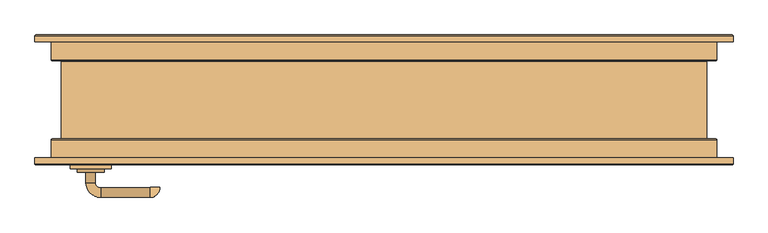
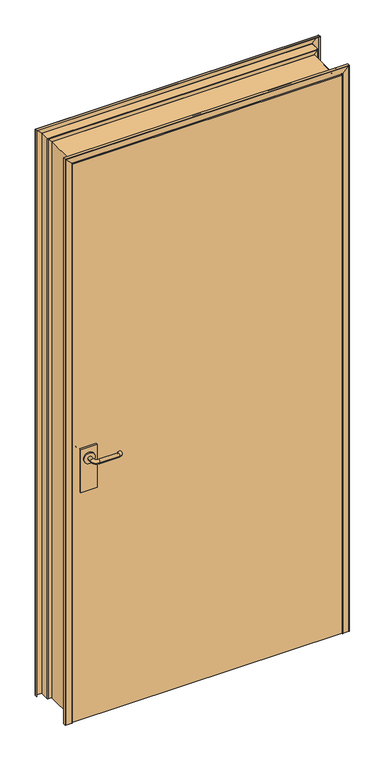
"""IFC4 building model written with IfcOpenShell, lengths in millimetres: door geometry, Porta Simples de Abrir : 90x210cm - Marco Metálico."""

from ifc_helpers import new_model, si_unit, point, frame, frame_2d, origin, place, context, project, spatial, polyline, circle_curve, ellipse_curve, trimmed, segment, composite_curve, outline, extrude, source, transform, mapped, element, save
from ifc_brep_helpers import plane_surface, cylinder_surface, revolved_surface, advanced_brep


def door_5cabed0b(model_context):
    return source(origin(), model_context, "Body", "SolidModel", [
        extrude(outline(composite_curve([segment(trimmed(circle_curve(frame_2d((1050.0, -432.0)), 20.0), [point((1050.0, -452.0))], [point((1050.0, -412.0))], False, "CARTESIAN"), True, "CONTINUOUS"), segment(trimmed(circle_curve(frame_2d((1050.0, -432.0)), 20.0), [point((1050.0, -412.0))], [point((1050.0, -452.0))], False, "CARTESIAN"), True, "CONTINUOUS")], self_intersect=False)), frame((0.0, -54.6, 0.0), z_axis=(0.0, 1.0, 0.0), x_axis=(0.0, 0.0, 1.0)), (0.0, 0.0, 1.0), 4.5929895),
        advanced_brep(
        [(-425.0, -50.0070105, 1050.0), (-439.0, -50.0070105, 1050.0), (-425.0, -34.6, 1050.0), (-439.0, -34.6, 1050.0), (-417.0, -12.6, 1050.0), (-417.0, -26.6, 1050.0), (-345.0, -26.6, 1050.0), (-345.0, -12.6, 1050.0), (-344.0, -27.6, 1050.0), (-330.0, -27.6, 1050.0)],
        [
            (0, 1, circle_curve(frame((-432.0, -50.0070105, 1050.0), z_axis=(0.0, -1.0, 0.0), x_axis=(-1.0, 0.0, 0.0)), 7.0)),
            (1, 0, circle_curve(frame((-432.0, -50.0070105, 1050.0), z_axis=(0.0, -1.0, 0.0), x_axis=(-1.0, 0.0, 0.0)), 7.0)),
            (0, 2),
            (2, 3, circle_curve(frame((-432.0, -34.6, 1050.0), z_axis=(0.0, -1.0, 0.0), x_axis=(-1.0, 0.0, 0.0)), 7.0)),
            (3, 1),
            (3, 2, circle_curve(frame((-432.0, -34.6, 1050.0), z_axis=(0.0, -1.0, 0.0), x_axis=(-1.0, 0.0, 0.0)), 7.0)),
            (4, 3, circle_curve(frame((-417.0, -34.6, 1050.0), z_axis=(0.0, 0.0, 1.0), x_axis=(-1.0, 0.0, 0.0)), 22.0)),
            (2, 5, circle_curve(frame((-417.0, -34.6, 1050.0), z_axis=(0.0, 0.0, -1.0), x_axis=(-1.0, 0.0, 0.0)), 8.0)),
            (5, 4, circle_curve(frame((-417.0, -19.6, 1050.0), z_axis=(-1.0, 0.0, 0.0), x_axis=(0.0, 1.0, 0.0)), 7.0)),
            (4, 5, circle_curve(frame((-417.0, -19.6, 1050.0), z_axis=(-1.0, 0.0, 0.0), x_axis=(0.0, 1.0, 0.0)), 7.0)),
            (5, 6),
            (6, 7, circle_curve(frame((-345.0, -19.6, 1050.0), z_axis=(-1.0, 0.0, 0.0), x_axis=(0.0, 1.0, 0.0)), 7.0)),
            (7, 4),
            (7, 6, circle_curve(frame((-345.0, -19.6, 1050.0), z_axis=(-1.0, 0.0, 0.0), x_axis=(0.0, 1.0, 0.0)), 7.0)),
            (8, 9, circle_curve(frame((-337.0, -27.6, 1050.0), z_axis=(0.0, -1.0, 0.0), x_axis=(1.0, 0.0, 0.0)), 7.0)),
            (9, 8, circle_curve(frame((-337.0, -27.6, 1050.0), z_axis=(0.0, -1.0, 0.0), x_axis=(1.0, 0.0, 0.0)), 7.0)),
            (9, 7, circle_curve(frame((-345.0, -27.6, 1050.0), z_axis=(0.0, 0.0, 1.0), x_axis=(0.0, 1.0, 0.0)), 15.0)),
            (6, 8, circle_curve(frame((-345.0, -27.6, 1050.0), z_axis=(0.0, 0.0, -1.0), x_axis=(0.0, 1.0, 0.0)), 1.0)),
        ],
        [
            plane_surface(frame((-432.0, -50.0070105, 1050.0), z_axis=(0.0, -1.0, 0.0), x_axis=(0.0, 0.0, 1.0))),
            cylinder_surface(frame((-432.0, -50.0070105, 1050.0), z_axis=(0.0, -1.0, 0.0), x_axis=(-1.0, 0.0, 0.0)), 7.0),
            revolved_surface(trimmed(ellipse_curve(frame((-432.0, -34.6, 1050.0), z_axis=(0.0, -1.0, 0.0), x_axis=(-1.0, 0.0, 0.0)), 7.0, 7.0), [point((-425.0, -34.6, 1050.0))], [point((-439.0, -34.6, 1050.0))], True, "CARTESIAN"), (-417.0, -34.6, 1050.0), (0.0, 0.0, -1.0)),
            revolved_surface(trimmed(ellipse_curve(frame((-432.0, -34.6, 1050.0), z_axis=(0.0, -1.0, 0.0), x_axis=(-1.0, 0.0, 0.0)), 7.0, 7.0), [point((-439.0, -34.6, 1050.0))], [point((-425.0, -34.6, 1050.0))], True, "CARTESIAN"), (-417.0, -34.6, 1050.0), (0.0, 0.0, -1.0)),
            cylinder_surface(frame((-417.0, -19.6, 1050.0), z_axis=(-1.0, 0.0, 0.0), x_axis=(0.0, 1.0, 0.0)), 7.0),
            plane_surface(frame((-337.0, -27.6, 1050.0), z_axis=(0.0, -1.0, 0.0), x_axis=(0.0, 0.0, 1.0))),
            revolved_surface(trimmed(ellipse_curve(frame((-345.0, -19.6, 1050.0), z_axis=(-1.0, 0.0, 0.0), x_axis=(0.0, 1.0, 0.0)), 7.0, 7.0), [point((-345.0, -26.6, 1050.0))], [point((-345.0, -12.6, 1050.0))], True, "CARTESIAN"), (-345.0, -27.6, 1050.0), (0.0, 0.0, -1.0)),
            revolved_surface(trimmed(ellipse_curve(frame((-345.0, -19.6, 1050.0), z_axis=(-1.0, 0.0, 0.0), x_axis=(0.0, 1.0, 0.0)), 7.0, 7.0), [point((-345.0, -12.6, 1050.0))], [point((-345.0, -26.6, 1050.0))], True, "CARTESIAN"), (-345.0, -27.6, 1050.0), (0.0, 0.0, -1.0)),
        ],
        [
            (0, [[1, 2]]),
            (1, [[-1, 3, 4, 5]]),
            (1, [[-2, -5, 6, -3]]),
            (2, [[7, -4, 8, 9]]),
            (3, [[-8, -6, -7, 10]]),
            (4, [[-9, 11, 12, 13]]),
            (4, [[-10, -13, 14, -11]]),
            (5, [[15, 16]]),
            (6, [[17, -12, 18, -16]]),
            (7, [[-18, -14, -17, -15]]),
        ],
    ),
        extrude(outline(polyline([(-402.0, -60.6), (-462.0, -60.6), (-462.0, -54.6), (-402.0, -54.6), (-402.0, -60.6)])), frame((0.0, 0.0, 925.0), z_axis=(0.0, 0.0, 1.0), x_axis=(1.0, 0.0, 0.0)), (0.0, 0.0, 1.0), 165.0),
        extrude(outline(composite_curve([segment(trimmed(circle_curve(frame_2d((1050.0, -432.0)), 20.0), [point((1050.0, -452.0))], [point((1050.0, -412.0))], False, "CARTESIAN"), True, "CONTINUOUS"), segment(trimmed(circle_curve(frame_2d((1050.0, -432.0)), 20.0), [point((1050.0, -412.0))], [point((1050.0, -452.0))], False, "CARTESIAN"), True, "CONTINUOUS")], self_intersect=False)), frame((0.0, -106.1929895, 0.0), z_axis=(0.0, 1.0, 0.0), x_axis=(0.0, 0.0, 1.0)), (0.0, 0.0, 1.0), 4.5929895),
        advanced_brep(
        [(-425.0, -106.1929895, 1050.0), (-439.0, -106.1929895, 1050.0), (-439.0, -121.6, 1050.0), (-425.0, -121.6, 1050.0), (-417.0, -143.6, 1050.0), (-417.0, -129.6, 1050.0), (-345.0, -143.6, 1050.0), (-345.0, -129.6, 1050.0), (-344.0, -128.6, 1050.0), (-330.0, -128.6, 1050.0)],
        [
            (0, 1, circle_curve(frame((-432.0, -106.1929895, 1050.0), z_axis=(0.0, 1.0, 0.0), x_axis=(-1.0, 0.0, 0.0)), 7.0)),
            (1, 0, circle_curve(frame((-432.0, -106.1929895, 1050.0), z_axis=(0.0, 1.0, 0.0), x_axis=(-1.0, 0.0, 0.0)), 7.0)),
            (1, 2),
            (2, 3, circle_curve(frame((-432.0, -121.6, 1050.0), z_axis=(0.0, 1.0, 0.0), x_axis=(-1.0, 0.0, 0.0)), 7.0)),
            (3, 0),
            (3, 2, circle_curve(frame((-432.0, -121.6, 1050.0), z_axis=(0.0, 1.0, 0.0), x_axis=(-1.0, 0.0, 0.0)), 7.0)),
            (4, 5, circle_curve(frame((-417.0, -136.6, 1050.0), z_axis=(-1.0, 0.0, 0.0), x_axis=(0.0, -1.0, 0.0)), 7.0)),
            (5, 3, circle_curve(frame((-417.0, -121.6, 1050.0), z_axis=(0.0, 0.0, -1.0), x_axis=(-1.0, 0.0, 0.0)), 8.0)),
            (2, 4, circle_curve(frame((-417.0, -121.6, 1050.0), z_axis=(0.0, 0.0, 1.0), x_axis=(-1.0, 0.0, 0.0)), 22.0)),
            (5, 4, circle_curve(frame((-417.0, -136.6, 1050.0), z_axis=(-1.0, 0.0, 0.0), x_axis=(0.0, -1.0, 0.0)), 7.0)),
            (4, 6),
            (6, 7, circle_curve(frame((-345.0, -136.6, 1050.0), z_axis=(-1.0, 0.0, 0.0), x_axis=(0.0, -1.0, 0.0)), 7.0)),
            (7, 5),
            (7, 6, circle_curve(frame((-345.0, -136.6, 1050.0), z_axis=(-1.0, 0.0, 0.0), x_axis=(0.0, -1.0, 0.0)), 7.0)),
            (8, 9, circle_curve(frame((-337.0, -128.6, 1050.0), z_axis=(0.0, 1.0, 0.0), x_axis=(1.0, 0.0, 0.0)), 7.0)),
            (9, 8, circle_curve(frame((-337.0, -128.6, 1050.0), z_axis=(0.0, 1.0, 0.0), x_axis=(1.0, 0.0, 0.0)), 7.0)),
            (8, 7, circle_curve(frame((-345.0, -128.6, 1050.0), z_axis=(0.0, 0.0, -1.0), x_axis=(0.0, -1.0, 0.0)), 1.0)),
            (6, 9, circle_curve(frame((-345.0, -128.6, 1050.0), z_axis=(0.0, 0.0, 1.0), x_axis=(0.0, -1.0, 0.0)), 15.0)),
        ],
        [
            plane_surface(frame((-432.0, -106.1929895, 1050.0), z_axis=(0.0, 1.0, 0.0), x_axis=(0.0, 0.0, 1.0))),
            cylinder_surface(frame((-432.0, -106.1929895, 1050.0), z_axis=(0.0, 1.0, 0.0), x_axis=(-1.0, 0.0, 0.0)), 7.0),
            revolved_surface(trimmed(ellipse_curve(frame((-432.0, -121.6, 1050.0), z_axis=(0.0, -1.0, 0.0), x_axis=(-1.0, 0.0, 0.0)), 7.0, 7.0), [point((-425.0, -121.6, 1050.0))], [point((-439.0, -121.6, 1050.0))], True, "CARTESIAN"), (-417.0, -121.6, 1050.0), (0.0, 0.0, -1.0)),
            revolved_surface(trimmed(ellipse_curve(frame((-432.0, -121.6, 1050.0), z_axis=(0.0, -1.0, 0.0), x_axis=(-1.0, 0.0, 0.0)), 7.0, 7.0), [point((-439.0, -121.6, 1050.0))], [point((-425.0, -121.6, 1050.0))], True, "CARTESIAN"), (-417.0, -121.6, 1050.0), (0.0, 0.0, -1.0)),
            cylinder_surface(frame((-417.0, -136.6, 1050.0), z_axis=(-1.0, 0.0, 0.0), x_axis=(0.0, -1.0, 0.0)), 7.0),
            plane_surface(frame((-337.0, -128.6, 1050.0), z_axis=(0.0, 1.0, 0.0), x_axis=(0.0, 0.0, 1.0))),
            revolved_surface(trimmed(ellipse_curve(frame((-345.0, -136.6, 1050.0), z_axis=(1.0, 0.0, 0.0), x_axis=(0.0, -1.0, 0.0)), 7.0, 7.0), [point((-345.0, -129.6, 1050.0))], [point((-345.0, -143.6, 1050.0))], True, "CARTESIAN"), (-345.0, -128.6, 1050.0), (0.0, 0.0, -1.0)),
            revolved_surface(trimmed(ellipse_curve(frame((-345.0, -136.6, 1050.0), z_axis=(1.0, 0.0, 0.0), x_axis=(0.0, -1.0, 0.0)), 7.0, 7.0), [point((-345.0, -143.6, 1050.0))], [point((-345.0, -129.6, 1050.0))], True, "CARTESIAN"), (-345.0, -128.6, 1050.0), (0.0, 0.0, -1.0)),
        ],
        [
            (0, [[1, 2]]),
            (1, [[3, 4, 5, -2]]),
            (1, [[-5, 6, -3, -1]]),
            (2, [[7, 8, -4, 9]]),
            (3, [[10, -9, -6, -8]]),
            (4, [[11, 12, 13, -7]]),
            (4, [[-13, 14, -11, -10]]),
            (5, [[15, 16]]),
            (6, [[-15, 17, -12, 18]]),
            (7, [[-16, -18, -14, -17]]),
        ],
    ),
        extrude(outline(polyline([(-402.0, -95.6), (-402.0, -101.6), (-462.0, -101.6), (-462.0, -95.6), (-402.0, -95.6)])), frame((0.0, 0.0, 925.0), z_axis=(0.0, 0.0, 1.0), x_axis=(1.0, 0.0, 0.0)), (0.0, 0.0, 1.0), 165.0),
        extrude(outline(polyline([(487.0, -60.6), (487.0, -95.6), (-487.0, -95.6), (-487.0, -60.6), (487.0, -60.6)])), frame((0.0, 0.0, 53.0), z_axis=(0.0, 0.0, 1.0), x_axis=(1.0, 0.0, 0.0)), (0.0, 0.0, 1.0), 2133.0),
        advanced_brep(
        [(-474.05, -57.1, 50.0), (-475.55, -58.6, 50.0), (-488.55, -58.6, 50.0), (-489.05, -59.1, 50.0), (-489.05, -94.1, 50.0), (-490.55, -95.6, 50.0), (-512.55, -95.6, 50.0), (-514.05, -94.1, 50.0), (-514.05, -85.6, 50.0), (-513.05, -85.6, 50.0), (-513.05, -94.1, 50.0), (-512.55, -94.6, 50.0), (-490.55, -94.6, 50.0), (-490.05, -94.1, 50.0), (-490.05, -59.1, 50.0), (-488.55, -57.6, 50.0), (-475.55, -57.6, 50.0), (-475.05, -57.1, 50.0), (-475.05, 57.1, 50.0), (-475.55, 57.6, 50.0), (-488.55, 57.6, 50.0), (-490.05, 59.1, 50.0), (-490.05, 94.1, 50.0), (-490.55, 94.6, 50.0), (-512.55, 94.6, 50.0), (-513.05, 94.1, 50.0), (-513.05, 85.6, 50.0), (-514.05, 85.6, 50.0), (-514.05, 94.1, 50.0), (-512.55, 95.6, 50.0), (-490.55, 95.6, 50.0), (-489.05, 94.1, 50.0), (-489.05, 59.1, 50.0), (-488.55, 58.6, 50.0), (-475.55, 58.6, 50.0), (-474.05, 57.1, 50.0), (-474.05, 57.1, 2174.05), (-474.05, -57.1, 2174.05), (-475.55, 58.6, 2175.55), (-488.55, 58.6, 2188.55), (-489.05, 59.1, 2189.05), (-489.05, 94.1, 2189.05), (-490.55, 95.6, 2190.55), (-512.55, 95.6, 2212.55), (-514.05, 94.1, 2214.05), (-514.05, 85.6, 2214.05), (-513.05, 85.6, 2213.05), (-513.05, 94.1, 2213.05), (-512.55, 94.6, 2212.55), (-490.55, 94.6, 2190.55), (-490.05, 94.1, 2190.05), (-490.05, 59.1, 2190.05), (-488.55, 57.6, 2188.55), (-475.55, 57.6, 2175.55), (-475.05, 57.1, 2175.05), (-475.05, -57.1, 2175.05), (-475.55, -57.6, 2175.55), (-488.55, -57.6, 2188.55), (-490.05, -59.1, 2190.05), (-490.05, -94.1, 2190.05), (-490.55, -94.6, 2190.55), (-512.55, -94.6, 2212.55), (-513.05, -94.1, 2213.05), (-513.05, -85.6, 2213.05), (-514.05, -85.6, 2214.05), (-514.05, -94.1, 2214.05), (-512.55, -95.6, 2212.55), (-490.55, -95.6, 2190.55), (-489.05, -94.1, 2189.05), (-489.05, -59.1, 2189.05), (-488.55, -58.6, 2188.55), (-475.55, -58.6, 2175.55), (474.05, -57.1, 50.0), (474.05, 57.1, 50.0), (475.55, 58.6, 50.0), (488.55, 58.6, 50.0), (489.05, 59.1, 50.0), (489.05, 94.1, 50.0), (490.55, 95.6, 50.0), (512.55, 95.6, 50.0), (514.05, 94.1, 50.0), (514.05, 85.6, 50.0), (513.05, 85.6, 50.0), (513.05, 94.1, 50.0), (512.55, 94.6, 50.0), (490.55, 94.6, 50.0), (490.05, 94.1, 50.0), (490.05, 59.1, 50.0), (488.55, 57.6, 50.0), (475.55, 57.6, 50.0), (475.05, 57.1, 50.0), (475.05, -57.1, 50.0), (475.55, -57.6, 50.0), (488.55, -57.6, 50.0), (490.05, -59.1, 50.0), (490.05, -94.1, 50.0), (490.55, -94.6, 50.0), (512.55, -94.6, 50.0), (513.05, -94.1, 50.0), (513.05, -85.6, 50.0), (514.05, -85.6, 50.0), (514.05, -94.1, 50.0), (512.55, -95.6, 50.0), (490.55, -95.6, 50.0), (489.05, -94.1, 50.0), (489.05, -59.1, 50.0), (488.55, -58.6, 50.0), (475.55, -58.6, 50.0), (474.05, -57.1, 2174.05), (475.55, -58.6, 2175.55), (488.55, -58.6, 2188.55), (489.05, -59.1, 2189.05), (489.05, -94.1, 2189.05), (490.55, -95.6, 2190.55), (512.55, -95.6, 2212.55), (514.05, -94.1, 2214.05), (514.05, -85.6, 2214.05), (513.05, -85.6, 2213.05), (513.05, -94.1, 2213.05), (512.55, -94.6, 2212.55), (490.55, -94.6, 2190.55), (490.05, -94.1, 2190.05), (490.05, -59.1, 2190.05), (488.55, -57.6, 2188.55), (475.55, -57.6, 2175.55), (475.05, -57.1, 2175.05), (475.05, 57.1, 2175.05), (475.55, 57.6, 2175.55), (488.55, 57.6, 2188.55), (490.05, 59.1, 2190.05), (490.05, 94.1, 2190.05), (490.55, 94.6, 2190.55), (512.55, 94.6, 2212.55), (513.05, 94.1, 2213.05), (513.05, 85.6, 2213.05), (514.05, 85.6, 2214.05), (514.05, 94.1, 2214.05), (512.55, 95.6, 2212.55), (490.55, 95.6, 2190.55), (489.05, 94.1, 2189.05), (489.05, 59.1, 2189.05), (488.55, 58.6, 2188.55), (475.55, 58.6, 2175.55), (474.05, 57.1, 2174.05)],
        [
            (0, 1, circle_curve(frame((-475.55, -57.1, 50.0), z_axis=(0.0, 0.0, -1.0), x_axis=(1.0, 0.0, 0.0)), 1.5)),
            (1, 2),
            (2, 3, circle_curve(frame((-488.55, -59.1, 50.0), z_axis=(0.0, 0.0, 1.0), x_axis=(1.0, 0.0, 0.0)), 0.5)),
            (3, 4),
            (4, 5, circle_curve(frame((-490.55, -94.1, 50.0), z_axis=(0.0, 0.0, -1.0), x_axis=(1.0, 0.0, 0.0)), 1.5)),
            (5, 6),
            (6, 7, circle_curve(frame((-512.55, -94.1, 50.0), z_axis=(0.0, 0.0, -1.0), x_axis=(1.0, 0.0, 0.0)), 1.5)),
            (7, 8),
            (8, 9),
            (9, 10),
            (10, 11, circle_curve(frame((-512.55, -94.1, 50.0), z_axis=(0.0, 0.0, 1.0), x_axis=(1.0, 0.0, 0.0)), 0.5)),
            (11, 12),
            (12, 13, circle_curve(frame((-490.55, -94.1, 50.0), z_axis=(0.0, 0.0, 1.0), x_axis=(1.0, 0.0, 0.0)), 0.5)),
            (13, 14),
            (14, 15, circle_curve(frame((-488.55, -59.1, 50.0), z_axis=(0.0, 0.0, -1.0), x_axis=(1.0, 0.0, 0.0)), 1.5)),
            (15, 16),
            (16, 17, circle_curve(frame((-475.55, -57.1, 50.0), z_axis=(0.0, 0.0, 1.0), x_axis=(1.0, 0.0, 0.0)), 0.5)),
            (17, 18),
            (18, 19, circle_curve(frame((-475.55, 57.1, 50.0), z_axis=(0.0, 0.0, 1.0), x_axis=(1.0, 0.0, 0.0)), 0.5)),
            (19, 20),
            (20, 21, circle_curve(frame((-488.55, 59.1, 50.0), z_axis=(0.0, 0.0, -1.0), x_axis=(1.0, 0.0, 0.0)), 1.5)),
            (21, 22),
            (22, 23, circle_curve(frame((-490.55, 94.1, 50.0), z_axis=(0.0, 0.0, 1.0), x_axis=(1.0, 0.0, 0.0)), 0.5)),
            (23, 24),
            (24, 25, circle_curve(frame((-512.55, 94.1, 50.0), z_axis=(0.0, 0.0, 1.0), x_axis=(1.0, 0.0, 0.0)), 0.5)),
            (25, 26),
            (26, 27),
            (27, 28),
            (28, 29, circle_curve(frame((-512.55, 94.1, 50.0), z_axis=(0.0, 0.0, -1.0), x_axis=(1.0, 0.0, 0.0)), 1.5)),
            (29, 30),
            (30, 31, circle_curve(frame((-490.55, 94.1, 50.0), z_axis=(0.0, 0.0, -1.0), x_axis=(1.0, 0.0, 0.0)), 1.5)),
            (31, 32),
            (32, 33, circle_curve(frame((-488.55, 59.1, 50.0), z_axis=(0.0, 0.0, 1.0), x_axis=(1.0, 0.0, 0.0)), 0.5)),
            (33, 34),
            (34, 35, circle_curve(frame((-475.55, 57.1, 50.0), z_axis=(0.0, 0.0, -1.0), x_axis=(1.0, 0.0, 0.0)), 1.5)),
            (35, 0),
            (35, 36),
            (36, 37),
            (37, 0),
            (34, 38),
            (38, 36, ellipse_curve(frame((-475.55, 57.1, 2175.55), z_axis=(-0.7071067811865475, 0.0, -0.7071067811865475), x_axis=(0.7071067811865474, 0.0, -0.7071067811865476)), 2.1213203, 1.5)),
            (33, 39),
            (39, 38),
            (32, 40),
            (40, 39, ellipse_curve(frame((-488.55, 59.1, 2188.55), z_axis=(0.7071067811865475, 0.0, 0.7071067811865475), x_axis=(-0.7071067811865474, 0.0, 0.7071067811865476)), 0.7071068, 0.5)),
            (31, 41),
            (41, 40),
            (30, 42),
            (42, 41, ellipse_curve(frame((-490.55, 94.1, 2190.55), z_axis=(-0.7071067811865475, 0.0, -0.7071067811865475), x_axis=(0.7071067811865474, 0.0, -0.7071067811865476)), 2.1213203, 1.5)),
            (29, 43),
            (43, 42),
            (28, 44),
            (44, 43, ellipse_curve(frame((-512.55, 94.1, 2212.55), z_axis=(-0.7071067811865475, 0.0, -0.7071067811865475), x_axis=(0.7071067811865474, 0.0, -0.7071067811865476)), 2.1213203, 1.5)),
            (27, 45),
            (45, 44),
            (26, 46),
            (46, 45),
            (25, 47),
            (47, 46),
            (24, 48),
            (48, 47, ellipse_curve(frame((-512.55, 94.1, 2212.55), z_axis=(0.7071067811865475, 0.0, 0.7071067811865475), x_axis=(-0.7071067811865474, 0.0, 0.7071067811865476)), 0.7071068, 0.5)),
            (23, 49),
            (49, 48),
            (22, 50),
            (50, 49, ellipse_curve(frame((-490.55, 94.1, 2190.55), z_axis=(0.7071067811865475, 0.0, 0.7071067811865475), x_axis=(-0.7071067811865474, 0.0, 0.7071067811865476)), 0.7071068, 0.5)),
            (21, 51),
            (51, 50),
            (20, 52),
            (52, 51, ellipse_curve(frame((-488.55, 59.1, 2188.55), z_axis=(-0.7071067811865475, 0.0, -0.7071067811865475), x_axis=(0.7071067811865474, 0.0, -0.7071067811865476)), 2.1213203, 1.5)),
            (19, 53),
            (53, 52),
            (18, 54),
            (54, 53, ellipse_curve(frame((-475.55, 57.1, 2175.55), z_axis=(0.7071067811865475, 0.0, 0.7071067811865475), x_axis=(-0.7071067811865474, 0.0, 0.7071067811865476)), 0.7071068, 0.5)),
            (17, 55),
            (55, 54),
            (16, 56),
            (56, 55, ellipse_curve(frame((-475.55, -57.1, 2175.55), z_axis=(0.7071067811865475, 0.0, 0.7071067811865475), x_axis=(-0.7071067811865474, 0.0, 0.7071067811865476)), 0.7071068, 0.5)),
            (15, 57),
            (57, 56),
            (14, 58),
            (58, 57, ellipse_curve(frame((-488.55, -59.1, 2188.55), z_axis=(-0.7071067811865475, 0.0, -0.7071067811865475), x_axis=(0.7071067811865474, 0.0, -0.7071067811865476)), 2.1213203, 1.5)),
            (13, 59),
            (59, 58),
            (12, 60),
            (60, 59, ellipse_curve(frame((-490.55, -94.1, 2190.55), z_axis=(0.7071067811865475, 0.0, 0.7071067811865475), x_axis=(-0.7071067811865474, 0.0, 0.7071067811865476)), 0.7071068, 0.5)),
            (11, 61),
            (61, 60),
            (10, 62),
            (62, 61, ellipse_curve(frame((-512.55, -94.1, 2212.55), z_axis=(0.7071067811865475, 0.0, 0.7071067811865475), x_axis=(-0.7071067811865474, 0.0, 0.7071067811865476)), 0.7071068, 0.5)),
            (9, 63),
            (63, 62),
            (8, 64),
            (64, 63),
            (7, 65),
            (65, 64),
            (6, 66),
            (66, 65, ellipse_curve(frame((-512.55, -94.1, 2212.55), z_axis=(-0.7071067811865475, 0.0, -0.7071067811865475), x_axis=(0.7071067811865474, 0.0, -0.7071067811865476)), 2.1213203, 1.5)),
            (5, 67),
            (67, 66),
            (4, 68),
            (68, 67, ellipse_curve(frame((-490.55, -94.1, 2190.55), z_axis=(-0.7071067811865475, 0.0, -0.7071067811865475), x_axis=(0.7071067811865474, 0.0, -0.7071067811865476)), 2.1213203, 1.5)),
            (3, 69),
            (69, 68),
            (2, 70),
            (70, 69, ellipse_curve(frame((-488.55, -59.1, 2188.55), z_axis=(0.7071067811865475, 0.0, 0.7071067811865475), x_axis=(-0.7071067811865474, 0.0, 0.7071067811865476)), 0.7071068, 0.5)),
            (1, 71),
            (71, 70),
            (37, 71, ellipse_curve(frame((-475.55, -57.1, 2175.55), z_axis=(-0.7071067811865475, 0.0, -0.7071067811865475), x_axis=(0.7071067811865474, 0.0, -0.7071067811865476)), 2.1213203, 1.5)),
            (72, 73),
            (73, 74, circle_curve(frame((475.55, 57.1, 50.0), z_axis=(0.0, 0.0, -1.0), x_axis=(-1.0, 0.0, 0.0)), 1.5)),
            (74, 75),
            (75, 76, circle_curve(frame((488.55, 59.1, 50.0), z_axis=(0.0, 0.0, 1.0), x_axis=(-1.0, 0.0, 0.0)), 0.5)),
            (76, 77),
            (77, 78, circle_curve(frame((490.55, 94.1, 50.0), z_axis=(0.0, 0.0, -1.0), x_axis=(-1.0, 0.0, 0.0)), 1.5)),
            (78, 79),
            (79, 80, circle_curve(frame((512.55, 94.1, 50.0), z_axis=(0.0, 0.0, -1.0), x_axis=(-1.0, 0.0, 0.0)), 1.5)),
            (80, 81),
            (81, 82),
            (82, 83),
            (83, 84, circle_curve(frame((512.55, 94.1, 50.0), z_axis=(0.0, 0.0, 1.0), x_axis=(-1.0, 0.0, 0.0)), 0.5)),
            (84, 85),
            (85, 86, circle_curve(frame((490.55, 94.1, 50.0), z_axis=(0.0, 0.0, 1.0), x_axis=(-1.0, 0.0, 0.0)), 0.5)),
            (86, 87),
            (87, 88, circle_curve(frame((488.55, 59.1, 50.0), z_axis=(0.0, 0.0, -1.0), x_axis=(-1.0, 0.0, 0.0)), 1.5)),
            (88, 89),
            (89, 90, circle_curve(frame((475.55, 57.1, 50.0), z_axis=(0.0, 0.0, 1.0), x_axis=(-1.0, 0.0, 0.0)), 0.5)),
            (90, 91),
            (91, 92, circle_curve(frame((475.55, -57.1, 50.0), z_axis=(0.0, 0.0, 1.0), x_axis=(-1.0, 0.0, 0.0)), 0.5)),
            (92, 93),
            (93, 94, circle_curve(frame((488.55, -59.1, 50.0), z_axis=(0.0, 0.0, -1.0), x_axis=(-1.0, 0.0, 0.0)), 1.5)),
            (94, 95),
            (95, 96, circle_curve(frame((490.55, -94.1, 50.0), z_axis=(0.0, 0.0, 1.0), x_axis=(-1.0, 0.0, 0.0)), 0.5)),
            (96, 97),
            (97, 98, circle_curve(frame((512.55, -94.1, 50.0), z_axis=(0.0, 0.0, 1.0), x_axis=(-1.0, 0.0, 0.0)), 0.5)),
            (98, 99),
            (99, 100),
            (100, 101),
            (101, 102, circle_curve(frame((512.55, -94.1, 50.0), z_axis=(0.0, 0.0, -1.0), x_axis=(-1.0, 0.0, 0.0)), 1.5)),
            (102, 103),
            (103, 104, circle_curve(frame((490.55, -94.1, 50.0), z_axis=(0.0, 0.0, -1.0), x_axis=(-1.0, 0.0, 0.0)), 1.5)),
            (104, 105),
            (105, 106, circle_curve(frame((488.55, -59.1, 50.0), z_axis=(0.0, 0.0, 1.0), x_axis=(-1.0, 0.0, 0.0)), 0.5)),
            (106, 107),
            (107, 72, circle_curve(frame((475.55, -57.1, 50.0), z_axis=(0.0, 0.0, -1.0), x_axis=(-1.0, 0.0, 0.0)), 1.5)),
            (108, 72),
            (107, 109),
            (109, 108, ellipse_curve(frame((475.55, -57.1, 2175.55), z_axis=(0.7071067811865475, 0.0, -0.7071067811865475), x_axis=(0.7071067811865474, 0.0, 0.7071067811865476)), 2.1213203, 1.5)),
            (106, 110),
            (110, 109),
            (105, 111),
            (111, 110, ellipse_curve(frame((488.55, -59.1, 2188.55), z_axis=(-0.7071067811865475, 0.0, 0.7071067811865475), x_axis=(-0.7071067811865474, 0.0, -0.7071067811865476)), 0.7071068, 0.5)),
            (104, 112),
            (112, 111),
            (103, 113),
            (113, 112, ellipse_curve(frame((490.55, -94.1, 2190.55), z_axis=(0.7071067811865475, 0.0, -0.7071067811865475), x_axis=(0.7071067811865474, 0.0, 0.7071067811865476)), 2.1213203, 1.5)),
            (102, 114),
            (114, 113),
            (101, 115),
            (115, 114, ellipse_curve(frame((512.55, -94.1, 2212.55), z_axis=(0.7071067811865475, 0.0, -0.7071067811865475), x_axis=(0.7071067811865474, 0.0, 0.7071067811865476)), 2.1213203, 1.5)),
            (100, 116),
            (116, 115),
            (99, 117),
            (117, 116),
            (98, 118),
            (118, 117),
            (97, 119),
            (119, 118, ellipse_curve(frame((512.55, -94.1, 2212.55), z_axis=(-0.7071067811865475, 0.0, 0.7071067811865475), x_axis=(-0.7071067811865474, 0.0, -0.7071067811865476)), 0.7071068, 0.5)),
            (96, 120),
            (120, 119),
            (95, 121),
            (121, 120, ellipse_curve(frame((490.55, -94.1, 2190.55), z_axis=(-0.7071067811865475, 0.0, 0.7071067811865475), x_axis=(-0.7071067811865474, 0.0, -0.7071067811865476)), 0.7071068, 0.5)),
            (94, 122),
            (122, 121),
            (93, 123),
            (123, 122, ellipse_curve(frame((488.55, -59.1, 2188.55), z_axis=(0.7071067811865475, 0.0, -0.7071067811865475), x_axis=(0.7071067811865474, 0.0, 0.7071067811865476)), 2.1213203, 1.5)),
            (92, 124),
            (124, 123),
            (91, 125),
            (125, 124, ellipse_curve(frame((475.55, -57.1, 2175.55), z_axis=(-0.7071067811865475, 0.0, 0.7071067811865475), x_axis=(-0.7071067811865474, 0.0, -0.7071067811865476)), 0.7071068, 0.5)),
            (90, 126),
            (126, 125),
            (89, 127),
            (127, 126, ellipse_curve(frame((475.55, 57.1, 2175.55), z_axis=(-0.7071067811865475, 0.0, 0.7071067811865475), x_axis=(-0.7071067811865474, 0.0, -0.7071067811865476)), 0.7071068, 0.5)),
            (88, 128),
            (128, 127),
            (87, 129),
            (129, 128, ellipse_curve(frame((488.55, 59.1, 2188.55), z_axis=(0.7071067811865475, 0.0, -0.7071067811865475), x_axis=(0.7071067811865474, 0.0, 0.7071067811865476)), 2.1213203, 1.5)),
            (86, 130),
            (130, 129),
            (85, 131),
            (131, 130, ellipse_curve(frame((490.55, 94.1, 2190.55), z_axis=(-0.7071067811865475, 0.0, 0.7071067811865475), x_axis=(-0.7071067811865474, 0.0, -0.7071067811865476)), 0.7071068, 0.5)),
            (84, 132),
            (132, 131),
            (83, 133),
            (133, 132, ellipse_curve(frame((512.55, 94.1, 2212.55), z_axis=(-0.7071067811865475, 0.0, 0.7071067811865475), x_axis=(-0.7071067811865474, 0.0, -0.7071067811865476)), 0.7071068, 0.5)),
            (82, 134),
            (134, 133),
            (81, 135),
            (135, 134),
            (80, 136),
            (136, 135),
            (79, 137),
            (137, 136, ellipse_curve(frame((512.55, 94.1, 2212.55), z_axis=(0.7071067811865475, 0.0, -0.7071067811865475), x_axis=(0.7071067811865474, 0.0, 0.7071067811865476)), 2.1213203, 1.5)),
            (78, 138),
            (138, 137),
            (77, 139),
            (139, 138, ellipse_curve(frame((490.55, 94.1, 2190.55), z_axis=(0.7071067811865475, 0.0, -0.7071067811865475), x_axis=(0.7071067811865474, 0.0, 0.7071067811865476)), 2.1213203, 1.5)),
            (76, 140),
            (140, 139),
            (75, 141),
            (141, 140, ellipse_curve(frame((488.55, 59.1, 2188.55), z_axis=(-0.7071067811865475, 0.0, 0.7071067811865475), x_axis=(-0.7071067811865474, 0.0, -0.7071067811865476)), 0.7071068, 0.5)),
            (74, 142),
            (142, 141),
            (73, 143),
            (143, 142, ellipse_curve(frame((475.55, 57.1, 2175.55), z_axis=(0.7071067811865475, 0.0, -0.7071067811865475), x_axis=(0.7071067811865474, 0.0, 0.7071067811865476)), 2.1213203, 1.5)),
            (108, 143),
            (36, 143),
            (108, 37),
            (38, 142),
            (39, 141),
            (40, 140),
            (41, 139),
            (42, 138),
            (43, 137),
            (44, 136),
            (45, 135),
            (46, 134),
            (47, 133),
            (48, 132),
            (49, 131),
            (50, 130),
            (51, 129),
            (52, 128),
            (53, 127),
            (54, 126),
            (55, 125),
            (56, 124),
            (57, 123),
            (58, 122),
            (59, 121),
            (60, 120),
            (61, 119),
            (62, 118),
            (63, 117),
            (64, 116),
            (65, 115),
            (66, 114),
            (67, 113),
            (68, 112),
            (69, 111),
            (70, 110),
            (71, 109),
        ],
        [
            plane_surface(frame((-500.0, 96.0340896, 50.0), z_axis=(0.0, 0.0, -1.0), x_axis=(1.0, 0.0, 0.0))),
            plane_surface(frame((-474.05, -57.1, 50.0), z_axis=(1.0, 0.0, 0.0), x_axis=(0.0, 0.0, 1.0))),
            cylinder_surface(frame((-475.55, 57.1, 50.0), z_axis=(0.0, 0.0, -1.0), x_axis=(1.0, 0.0, 0.0)), 1.5),
            plane_surface(frame((-475.55, 58.6, 50.0), z_axis=(0.0, 1.0, 0.0), x_axis=(0.0, 0.0, 1.0))),
            revolved_surface(polyline([(-488.05, 59.1, 2189.0500000133034), (-488.05, 59.1, 50.0)]), (-488.55, 59.1, 50.0), (0.0, 0.0, 1.0)),
            plane_surface(frame((-489.05, 59.1, 50.0), z_axis=(1.0, 0.0, 0.0), x_axis=(0.0, 0.0, 1.0))),
            cylinder_surface(frame((-490.55, 94.1, 50.0), z_axis=(0.0, 0.0, -1.0), x_axis=(1.0, 0.0, 0.0)), 1.5),
            plane_surface(frame((-490.55, 95.6, 50.0), z_axis=(0.0, 1.0, 0.0), x_axis=(0.0, 0.0, 1.0))),
            cylinder_surface(frame((-512.55, 94.1, 50.0), z_axis=(0.0, 0.0, -1.0), x_axis=(1.0, 0.0, 0.0)), 1.5),
            plane_surface(frame((-514.05, 94.1, 50.0), z_axis=(-1.0, 0.0, 0.0), x_axis=(0.0, 0.0, 1.0))),
            plane_surface(frame((-514.05, 85.6, 50.0), z_axis=(0.0, -1.0, 0.0), x_axis=(0.0, 0.0, 1.0))),
            plane_surface(frame((-513.05, 85.6, 50.0), z_axis=(1.0, 0.0, 0.0), x_axis=(0.0, 0.0, 1.0))),
            revolved_surface(polyline([(-512.05, 94.1, 2213.0500000133034), (-512.05, 94.1, 50.0)]), (-512.55, 94.1, 50.0), (0.0, 0.0, 1.0)),
            plane_surface(frame((-512.55, 94.6, 50.0), z_axis=(0.0, -1.0, 0.0), x_axis=(0.0, 0.0, 1.0))),
            revolved_surface(polyline([(-490.05, 94.1, 2191.0500000133034), (-490.05, 94.1, 50.0)]), (-490.55, 94.1, 50.0), (0.0, 0.0, 1.0)),
            plane_surface(frame((-490.05, 94.1, 50.0), z_axis=(-1.0, 0.0, 0.0), x_axis=(0.0, 0.0, 1.0))),
            cylinder_surface(frame((-488.55, 59.1, 50.0), z_axis=(0.0, 0.0, -1.0), x_axis=(1.0, 0.0, 0.0)), 1.5),
            plane_surface(frame((-488.55, 57.6, 50.0), z_axis=(0.0, -1.0, 0.0), x_axis=(0.0, 0.0, 1.0))),
            revolved_surface(polyline([(-475.05, 57.1, 2176.0500000133034), (-475.05, 57.1, 50.0)]), (-475.55, 57.1, 50.0), (0.0, 0.0, 1.0)),
            plane_surface(frame((-475.05, 57.1, 50.0), z_axis=(-1.0, 0.0, 0.0), x_axis=(0.0, 0.0, 1.0))),
            revolved_surface(polyline([(-475.05, -57.1, 2176.0500000133034), (-475.05, -57.1, 50.0)]), (-475.55, -57.1, 50.0), (0.0, 0.0, 1.0)),
            plane_surface(frame((-475.55, -57.6, 50.0), z_axis=(0.0, 1.0, 0.0), x_axis=(0.0, 0.0, 1.0))),
            cylinder_surface(frame((-488.55, -59.1, 50.0), z_axis=(0.0, 0.0, -1.0), x_axis=(1.0, 0.0, 0.0)), 1.5),
            plane_surface(frame((-490.05, -59.1, 50.0), z_axis=(-1.0, 0.0, 0.0), x_axis=(0.0, 0.0, 1.0))),
            revolved_surface(polyline([(-490.05, -94.1, 2191.0500000133034), (-490.05, -94.1, 50.0)]), (-490.55, -94.1, 50.0), (0.0, 0.0, 1.0)),
            plane_surface(frame((-490.55, -94.6, 50.0), z_axis=(0.0, 1.0, 0.0), x_axis=(0.0, 0.0, 1.0))),
            revolved_surface(polyline([(-512.05, -94.1, 2213.0500000133034), (-512.05, -94.1, 50.0)]), (-512.55, -94.1, 50.0), (0.0, 0.0, 1.0)),
            plane_surface(frame((-513.05, -94.1, 50.0), z_axis=(1.0, 0.0, 0.0), x_axis=(0.0, 0.0, 1.0))),
            plane_surface(frame((-513.05, -85.6, 50.0), z_axis=(0.0, 1.0, 0.0), x_axis=(0.0, 0.0, 1.0))),
            plane_surface(frame((-514.05, -85.6, 50.0), z_axis=(-1.0, 0.0, 0.0), x_axis=(0.0, 0.0, 1.0))),
            cylinder_surface(frame((-512.55, -94.1, 50.0), z_axis=(0.0, 0.0, -1.0), x_axis=(1.0, 0.0, 0.0)), 1.5),
            plane_surface(frame((-512.55, -95.6, 50.0), z_axis=(0.0, -1.0, 0.0), x_axis=(0.0, 0.0, 1.0))),
            cylinder_surface(frame((-490.55, -94.1, 50.0), z_axis=(0.0, 0.0, -1.0), x_axis=(1.0, 0.0, 0.0)), 1.5),
            plane_surface(frame((-489.05, -94.1, 50.0), z_axis=(1.0, 0.0, 0.0), x_axis=(0.0, 0.0, 1.0))),
            revolved_surface(polyline([(-488.05, -59.1, 2189.0500000133034), (-488.05, -59.1, 50.0)]), (-488.55, -59.1, 50.0), (0.0, 0.0, 1.0)),
            plane_surface(frame((-488.55, -58.6, 50.0), z_axis=(0.0, -1.0, 0.0), x_axis=(0.0, 0.0, 1.0))),
            cylinder_surface(frame((-475.55, -57.1, 50.0), z_axis=(0.0, 0.0, -1.0), x_axis=(1.0, 0.0, 0.0)), 1.5),
            plane_surface(frame((500.0, 96.0340896, 50.0), z_axis=(0.0, 0.0, -1.0), x_axis=(-1.0, 0.0, 0.0))),
            cylinder_surface(frame((475.55, -57.1, 2200.0), z_axis=(0.0, 0.0, 1.0), x_axis=(-1.0, 0.0, 0.0)), 1.5),
            plane_surface(frame((488.55, -58.6, 2188.55), z_axis=(0.0, -1.0, 0.0), x_axis=(0.0, 0.0, -1.0))),
            revolved_surface(polyline([(488.05, -59.1, 50.0), (488.05, -59.1, 2189.0500000133034)]), (488.55, -59.1, 2200.0), (0.0, 0.0, -1.0)),
            plane_surface(frame((489.05, -94.1, 2189.05), z_axis=(-1.0, 0.0, 0.0), x_axis=(0.0, 0.0, -1.0))),
            cylinder_surface(frame((490.55, -94.1, 2200.0), z_axis=(0.0, 0.0, 1.0), x_axis=(-1.0, 0.0, 0.0)), 1.5),
            plane_surface(frame((512.55, -95.6, 2212.55), z_axis=(0.0, -1.0, 0.0), x_axis=(0.0, 0.0, -1.0))),
            cylinder_surface(frame((512.55, -94.1, 2200.0), z_axis=(0.0, 0.0, 1.0), x_axis=(-1.0, 0.0, 0.0)), 1.5),
            plane_surface(frame((514.05, -85.6, 2214.05), z_axis=(1.0, 0.0, 0.0), x_axis=(0.0, 0.0, -1.0))),
            plane_surface(frame((513.05, -85.6, 2213.05), z_axis=(0.0, 1.0, 0.0), x_axis=(0.0, 0.0, -1.0))),
            plane_surface(frame((513.05, -94.1, 2213.05), z_axis=(-1.0, 0.0, 0.0), x_axis=(0.0, 0.0, -1.0))),
            revolved_surface(polyline([(512.05, -94.1, 50.0), (512.05, -94.1, 2213.0500000133034)]), (512.55, -94.1, 2200.0), (0.0, 0.0, -1.0)),
            plane_surface(frame((490.55, -94.6, 2190.55), z_axis=(0.0, 1.0, 0.0), x_axis=(0.0, 0.0, -1.0))),
            revolved_surface(polyline([(490.05, -94.1, 50.0), (490.05, -94.1, 2191.0500000133034)]), (490.55, -94.1, 2200.0), (0.0, 0.0, -1.0)),
            plane_surface(frame((490.05, -59.1, 2190.05), z_axis=(1.0, 0.0, 0.0), x_axis=(0.0, 0.0, -1.0))),
            cylinder_surface(frame((488.55, -59.1, 2200.0), z_axis=(0.0, 0.0, 1.0), x_axis=(-1.0, 0.0, 0.0)), 1.5),
            plane_surface(frame((475.55, -57.6, 2175.55), z_axis=(0.0, 1.0, 0.0), x_axis=(0.0, 0.0, -1.0))),
            revolved_surface(polyline([(475.05, -57.1, 50.0), (475.05, -57.1, 2176.0500000133034)]), (475.55, -57.1, 2200.0), (0.0, 0.0, -1.0)),
            plane_surface(frame((475.05, 57.1, 2175.05), z_axis=(1.0, 0.0, 0.0), x_axis=(0.0, 0.0, -1.0))),
            revolved_surface(polyline([(475.05, 57.1, 50.0), (475.05, 57.1, 2176.0500000133034)]), (475.55, 57.1, 2200.0), (0.0, 0.0, -1.0)),
            plane_surface(frame((488.55, 57.6, 2188.55), z_axis=(0.0, -1.0, 0.0), x_axis=(0.0, 0.0, -1.0))),
            cylinder_surface(frame((488.55, 59.1, 2200.0), z_axis=(0.0, 0.0, 1.0), x_axis=(-1.0, 0.0, 0.0)), 1.5),
            plane_surface(frame((490.05, 94.1, 2190.05), z_axis=(1.0, 0.0, 0.0), x_axis=(0.0, 0.0, -1.0))),
            revolved_surface(polyline([(490.05, 94.1, 50.0), (490.05, 94.1, 2191.0500000133034)]), (490.55, 94.1, 2200.0), (0.0, 0.0, -1.0)),
            plane_surface(frame((512.55, 94.6, 2212.55), z_axis=(0.0, -1.0, 0.0), x_axis=(0.0, 0.0, -1.0))),
            revolved_surface(polyline([(512.05, 94.1, 50.0), (512.05, 94.1, 2213.0500000133034)]), (512.55, 94.1, 2200.0), (0.0, 0.0, -1.0)),
            plane_surface(frame((513.05, 85.6, 2213.05), z_axis=(-1.0, 0.0, 0.0), x_axis=(0.0, 0.0, -1.0))),
            plane_surface(frame((514.05, 85.6, 2214.05), z_axis=(0.0, -1.0, 0.0), x_axis=(0.0, 0.0, -1.0))),
            plane_surface(frame((514.05, 94.1, 2214.05), z_axis=(1.0, 0.0, 0.0), x_axis=(0.0, 0.0, -1.0))),
            cylinder_surface(frame((512.55, 94.1, 2200.0), z_axis=(0.0, 0.0, 1.0), x_axis=(-1.0, 0.0, 0.0)), 1.5),
            plane_surface(frame((490.55, 95.6, 2190.55), z_axis=(0.0, 1.0, 0.0), x_axis=(0.0, 0.0, -1.0))),
            cylinder_surface(frame((490.55, 94.1, 2200.0), z_axis=(0.0, 0.0, 1.0), x_axis=(-1.0, 0.0, 0.0)), 1.5),
            plane_surface(frame((489.05, 59.1, 2189.05), z_axis=(-1.0, 0.0, 0.0), x_axis=(0.0, 0.0, -1.0))),
            revolved_surface(polyline([(488.05, 59.1, 50.0), (488.05, 59.1, 2189.0500000133034)]), (488.55, 59.1, 2200.0), (0.0, 0.0, -1.0)),
            plane_surface(frame((475.55, 58.6, 2175.55), z_axis=(0.0, 1.0, 0.0), x_axis=(0.0, 0.0, -1.0))),
            cylinder_surface(frame((475.55, 57.1, 2200.0), z_axis=(0.0, 0.0, 1.0), x_axis=(-1.0, 0.0, 0.0)), 1.5),
            plane_surface(frame((474.05, -57.1, 2174.05), z_axis=(-1.0, 0.0, 0.0), x_axis=(0.0, 0.0, -1.0))),
            plane_surface(frame((-474.05, -57.1, 2174.05), z_axis=(0.0, 0.0, -1.0), x_axis=(1.0, 0.0, 0.0))),
            cylinder_surface(frame((-500.0, 57.1, 2175.55), z_axis=(-1.0, 0.0, 0.0), x_axis=(0.0, 0.0, -1.0)), 1.5),
            plane_surface(frame((-475.55, 58.6, 2175.55), z_axis=(0.0, 1.0, 0.0), x_axis=(1.0, 0.0, 0.0))),
            revolved_surface(polyline([(489.050000013303, 59.1, 2188.05), (-489.05000001330313, 59.1, 2188.05)]), (-500.0, 59.1, 2188.55), (1.0, 0.0, 0.0)),
            plane_surface(frame((-489.05, 59.1, 2189.05), z_axis=(0.0, 0.0, -1.0), x_axis=(1.0, 0.0, 0.0))),
            cylinder_surface(frame((-500.0, 94.1, 2190.55), z_axis=(-1.0, 0.0, 0.0), x_axis=(0.0, 0.0, -1.0)), 1.5),
            plane_surface(frame((-490.55, 95.6, 2190.55), z_axis=(0.0, 1.0, 0.0), x_axis=(1.0, 0.0, 0.0))),
            cylinder_surface(frame((-500.0, 94.1, 2212.55), z_axis=(-1.0, 0.0, 0.0), x_axis=(0.0, 0.0, -1.0)), 1.5),
            plane_surface(frame((-514.05, 94.1, 2214.05), z_axis=(0.0, 0.0, 1.0), x_axis=(1.0, 0.0, 0.0))),
            plane_surface(frame((-514.05, 85.6, 2214.05), z_axis=(0.0, -1.0, 0.0), x_axis=(1.0, 0.0, 0.0))),
            plane_surface(frame((-513.05, 85.6, 2213.05), z_axis=(0.0, 0.0, -1.0), x_axis=(1.0, 0.0, 0.0))),
            revolved_surface(polyline([(513.050000013303, 94.1, 2212.05), (-513.050000013303, 94.1, 2212.05)]), (-500.0, 94.1, 2212.55), (1.0, 0.0, 0.0)),
            plane_surface(frame((-512.55, 94.6, 2212.55), z_axis=(0.0, -1.0, 0.0), x_axis=(1.0, 0.0, 0.0))),
            revolved_surface(polyline([(491.050000013303, 94.1, 2190.05), (-491.05000001330313, 94.1, 2190.05)]), (-500.0, 94.1, 2190.55), (1.0, 0.0, 0.0)),
            plane_surface(frame((-490.05, 94.1, 2190.05), z_axis=(0.0, 0.0, 1.0), x_axis=(1.0, 0.0, 0.0))),
            cylinder_surface(frame((-500.0, 59.1, 2188.55), z_axis=(-1.0, 0.0, 0.0), x_axis=(0.0, 0.0, -1.0)), 1.5),
            plane_surface(frame((-488.55, 57.6, 2188.55), z_axis=(0.0, -1.0, 0.0), x_axis=(1.0, 0.0, 0.0))),
            revolved_surface(polyline([(476.050000013303, 57.1, 2175.05), (-476.05000001330313, 57.1, 2175.05)]), (-500.0, 57.1, 2175.55), (1.0, 0.0, 0.0)),
            plane_surface(frame((-475.05, 57.1, 2175.05), z_axis=(0.0, 0.0, 1.0), x_axis=(1.0, 0.0, 0.0))),
            revolved_surface(polyline([(476.050000013303, -57.1, 2175.05), (-476.05000001330313, -57.1, 2175.05)]), (-500.0, -57.1, 2175.55), (1.0, 0.0, 0.0)),
            plane_surface(frame((-475.55, -57.6, 2175.55), z_axis=(0.0, 1.0, 0.0), x_axis=(1.0, 0.0, 0.0))),
            cylinder_surface(frame((-500.0, -59.1, 2188.55), z_axis=(-1.0, 0.0, 0.0), x_axis=(0.0, 0.0, -1.0)), 1.5),
            plane_surface(frame((-490.05, -59.1, 2190.05), z_axis=(0.0, 0.0, 1.0), x_axis=(1.0, 0.0, 0.0))),
            revolved_surface(polyline([(491.050000013303, -94.1, 2190.05), (-491.05000001330313, -94.1, 2190.05)]), (-500.0, -94.1, 2190.55), (1.0, 0.0, 0.0)),
            plane_surface(frame((-490.55, -94.6, 2190.55), z_axis=(0.0, 1.0, 0.0), x_axis=(1.0, 0.0, 0.0))),
            revolved_surface(polyline([(513.050000013303, -94.1, 2212.05), (-513.050000013303, -94.1, 2212.05)]), (-500.0, -94.1, 2212.55), (1.0, 0.0, 0.0)),
            plane_surface(frame((-513.05, -94.1, 2213.05), z_axis=(0.0, 0.0, -1.0), x_axis=(1.0, 0.0, 0.0))),
            plane_surface(frame((-513.05, -85.6, 2213.05), z_axis=(0.0, 1.0, 0.0), x_axis=(1.0, 0.0, 0.0))),
            plane_surface(frame((-514.05, -85.6, 2214.05), z_axis=(0.0, 0.0, 1.0), x_axis=(1.0, 0.0, 0.0))),
            cylinder_surface(frame((-500.0, -94.1, 2212.55), z_axis=(-1.0, 0.0, 0.0), x_axis=(0.0, 0.0, -1.0)), 1.5),
            plane_surface(frame((-512.55, -95.6, 2212.55), z_axis=(0.0, -1.0, 0.0), x_axis=(1.0, 0.0, 0.0))),
            cylinder_surface(frame((-500.0, -94.1, 2190.55), z_axis=(-1.0, 0.0, 0.0), x_axis=(0.0, 0.0, -1.0)), 1.5),
            plane_surface(frame((-489.05, -94.1, 2189.05), z_axis=(0.0, 0.0, -1.0), x_axis=(1.0, 0.0, 0.0))),
            revolved_surface(polyline([(489.050000013303, -59.1, 2188.05), (-489.05000001330313, -59.1, 2188.05)]), (-500.0, -59.1, 2188.55), (1.0, 0.0, 0.0)),
            plane_surface(frame((-488.55, -58.6, 2188.55), z_axis=(0.0, -1.0, 0.0), x_axis=(1.0, 0.0, 0.0))),
            cylinder_surface(frame((-500.0, -57.1, 2175.55), z_axis=(-1.0, 0.0, 0.0), x_axis=(0.0, 0.0, -1.0)), 1.5),
        ],
        [
            (0, [[1, 2, 3, 4, 5, 6, 7, 8, 9, 10, 11, 12, 13, 14, 15, 16, 17, 18, 19, 20, 21, 22, 23, 24, 25, 26, 27, 28, 29, 30, 31, 32, 33, 34, 35, 36]]),
            (1, [[37, 38, 39, -36]]),
            (2, [[40, 41, -37, -35]]),
            (3, [[42, 43, -40, -34]]),
            (4, [[44, 45, -42, -33]]),
            (5, [[46, 47, -44, -32]]),
            (6, [[48, 49, -46, -31]]),
            (7, [[50, 51, -48, -30]]),
            (8, [[52, 53, -50, -29]]),
            (9, [[54, 55, -52, -28]]),
            (10, [[56, 57, -54, -27]]),
            (11, [[58, 59, -56, -26]]),
            (12, [[60, 61, -58, -25]]),
            (13, [[62, 63, -60, -24]]),
            (14, [[64, 65, -62, -23]]),
            (15, [[66, 67, -64, -22]]),
            (16, [[68, 69, -66, -21]]),
            (17, [[70, 71, -68, -20]]),
            (18, [[72, 73, -70, -19]]),
            (19, [[74, 75, -72, -18]]),
            (20, [[76, 77, -74, -17]]),
            (21, [[78, 79, -76, -16]]),
            (22, [[80, 81, -78, -15]]),
            (23, [[82, 83, -80, -14]]),
            (24, [[84, 85, -82, -13]]),
            (25, [[86, 87, -84, -12]]),
            (26, [[88, 89, -86, -11]]),
            (27, [[90, 91, -88, -10]]),
            (28, [[92, 93, -90, -9]]),
            (29, [[94, 95, -92, -8]]),
            (30, [[96, 97, -94, -7]]),
            (31, [[98, 99, -96, -6]]),
            (32, [[100, 101, -98, -5]]),
            (33, [[102, 103, -100, -4]]),
            (34, [[104, 105, -102, -3]]),
            (35, [[106, 107, -104, -2]]),
            (36, [[-39, 108, -106, -1]]),
            (37, [[109, 110, 111, 112, 113, 114, 115, 116, 117, 118, 119, 120, 121, 122, 123, 124, 125, 126, 127, 128, 129, 130, 131, 132, 133, 134, 135, 136, 137, 138, 139, 140, 141, 142, 143, 144]]),
            (38, [[145, -144, 146, 147]]),
            (39, [[-146, -143, 148, 149]]),
            (40, [[-148, -142, 150, 151]]),
            (41, [[-150, -141, 152, 153]]),
            (42, [[-152, -140, 154, 155]]),
            (43, [[-154, -139, 156, 157]]),
            (44, [[-156, -138, 158, 159]]),
            (45, [[-158, -137, 160, 161]]),
            (46, [[-160, -136, 162, 163]]),
            (47, [[-162, -135, 164, 165]]),
            (48, [[-164, -134, 166, 167]]),
            (49, [[-166, -133, 168, 169]]),
            (50, [[-168, -132, 170, 171]]),
            (51, [[-170, -131, 172, 173]]),
            (52, [[-172, -130, 174, 175]]),
            (53, [[-174, -129, 176, 177]]),
            (54, [[-176, -128, 178, 179]]),
            (55, [[-178, -127, 180, 181]]),
            (56, [[-180, -126, 182, 183]]),
            (57, [[-182, -125, 184, 185]]),
            (58, [[-184, -124, 186, 187]]),
            (59, [[-186, -123, 188, 189]]),
            (60, [[-188, -122, 190, 191]]),
            (61, [[-190, -121, 192, 193]]),
            (62, [[-192, -120, 194, 195]]),
            (63, [[-194, -119, 196, 197]]),
            (64, [[-196, -118, 198, 199]]),
            (65, [[-198, -117, 200, 201]]),
            (66, [[-200, -116, 202, 203]]),
            (67, [[-202, -115, 204, 205]]),
            (68, [[-204, -114, 206, 207]]),
            (69, [[-206, -113, 208, 209]]),
            (70, [[-208, -112, 210, 211]]),
            (71, [[-210, -111, 212, 213]]),
            (72, [[-212, -110, 214, 215]]),
            (73, [[-214, -109, -145, 216]]),
            (74, [[217, -216, 218, -38]]),
            (75, [[219, -215, -217, -41]]),
            (76, [[220, -213, -219, -43]]),
            (77, [[221, -211, -220, -45]]),
            (78, [[222, -209, -221, -47]]),
            (79, [[223, -207, -222, -49]]),
            (80, [[224, -205, -223, -51]]),
            (81, [[225, -203, -224, -53]]),
            (82, [[226, -201, -225, -55]]),
            (83, [[227, -199, -226, -57]]),
            (84, [[228, -197, -227, -59]]),
            (85, [[229, -195, -228, -61]]),
            (86, [[230, -193, -229, -63]]),
            (87, [[231, -191, -230, -65]]),
            (88, [[232, -189, -231, -67]]),
            (89, [[233, -187, -232, -69]]),
            (90, [[234, -185, -233, -71]]),
            (91, [[235, -183, -234, -73]]),
            (92, [[236, -181, -235, -75]]),
            (93, [[237, -179, -236, -77]]),
            (94, [[238, -177, -237, -79]]),
            (95, [[239, -175, -238, -81]]),
            (96, [[240, -173, -239, -83]]),
            (97, [[241, -171, -240, -85]]),
            (98, [[242, -169, -241, -87]]),
            (99, [[243, -167, -242, -89]]),
            (100, [[244, -165, -243, -91]]),
            (101, [[245, -163, -244, -93]]),
            (102, [[246, -161, -245, -95]]),
            (103, [[247, -159, -246, -97]]),
            (104, [[248, -157, -247, -99]]),
            (105, [[249, -155, -248, -101]]),
            (106, [[250, -153, -249, -103]]),
            (107, [[251, -151, -250, -105]]),
            (108, [[252, -149, -251, -107]]),
            (109, [[-218, -147, -252, -108]]),
        ],
    ),
    ])


if __name__ == "__main__":
    model = new_model("IFC4")
    model_context = context("Model", 3, world=origin())
    ifc_project = project(units=[si_unit("LENGTHUNIT", "METRE", prefix="MILLI")], contexts=[model_context])
    site = spatial("IfcSite", under=ifc_project)
    building = spatial("IfcBuilding", under=site)
    placement = place(None, origin())
    door_shape = door_5cabed0b(model_context)
    element("IfcDoor", 1, ObjectType="Porta Simples de Abrir : 90x210cm - Marco Metálico", at=placement, inside=building, context=model_context, shape_type="MappedRepresentation", body=[
        mapped(door_shape, transform((0.0, 0.0, 0.0), x_axis=(1.0, 0.0, 0.0), y_axis=(0.0, 1.0, 0.0), z_axis=(0.0, 0.0, 1.0))),
    ])
    save(model, "model.ifc")

# Revit data of these elements
# Type "Porta Simples de Abrir : 90x210cm - Marco Metálico"
#   Type Mark = ""
#   SINAPI = ""
#   Construction Type = "300"
#   Maçaneta [instance default] = ""
#   Fechadura [instance default] = ""
#   Vão Luz (somente para informação) = 94.80 cm
#   Tolerância Folha Vertical = 0.30 cm
#   Módulo Básico M = 10.00 cm
#   Largura de Coordenação Modular Largura CM = 100.00 cm
#   Rough Width = 100.00 cm
#   Deslocamento da Horizontal da Folha = 1.00 cm
#   Altura de Coordenação Modular Largura CM = 220.00 cm
#   Rough Height = 220.00 cm
#   Altura Nominal = 212.40 cm
#   Ajuste de Coordenação Topo AC Topo = 0.00 cm
#   Ajuste de Coordenação Base AC Base = 5.00 cm
#   Ajuste de Coordenação AC = 0.00 cm
#   Tolerância Folha Horizontal = 0.20 cm
#   Largura Folha (somente para informação) = 97.40 cm
#   Espessura Folha = 3.50 cm
#   Maçaneta - Distância da Folha = 5.50 cm
#   Maçaneta - Altura = 100.00 cm
#   Largura Nominal (Largura Mn) = 97.80 cm
#   Distância do Nível = 0.30 cm
#   Aduela Interna Espessura = 1.10 cm
#   Aduela Externa Espessura = 2.60 cm
#   Altura Folha (somente para informação) = 211.90 cm
#   Height = 215.00 cm
#   Width = 100.00 cm
#   Número de Módulos Básicos nM Largura = 10
#   Número de Módulos Básicos nM Altura = 22
#   Marco Metálico = yes
#   Aduela de Madeira = no
#   Aduela Metálica de Canto = no
#   Guarnição Reta = no
#   Guarnição Chanfrada = no
#   Batente - Material [instance default] = none
#   Painel - Material [instance default] = none
#   Model = ""
#   Function = (empty or 0)
#   Description = (empty or 0)
#   Wall Closure = (empty or 0)
#   Assembly Code = ""
# Element 1 (IfcDoor, "Porta Simples de Abrir : 90x210cm - Marco Metálico")
#   Materials on its faces: "Porta - Maçaneta"
# Materials
#   "Porta - Maçaneta": class "Metal", colour RGB 189 187 185, transparency 0, Cost = 0
